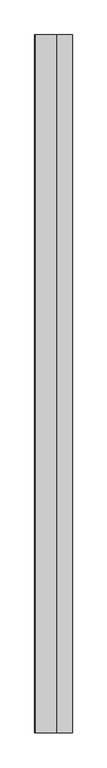
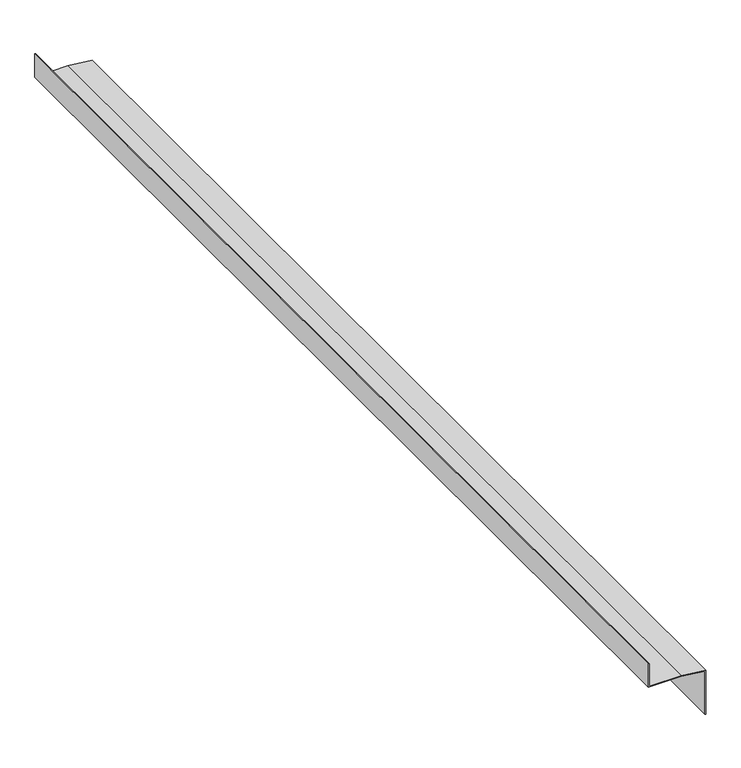
"""IFC4 building model written with IfcOpenShell, lengths in millimetres: proxy geometry, Generic Models 7:Generic Models 1:7:Generic Models 1:7 : Generic Models 7:Generic Models 1:337419:8 : Generic Models 7:Generic Models 1:7:Generic Models 1:7 : Generic Models 7:Generic Models 1:337419:315055."""

from ifc_helpers import new_model, si_unit, frame, origin, place, context, project, spatial, polyline, outline, extrude, source, transform, mapped, element, save


def generic_models_aac07dfa(model_context):
    return source(origin(), model_context, "Body", "SweptSolid", [
        extrude(outline(polyline([(-1.5875, 0.0), (0.0, 0.0), (0.0, -106.0492371), (-55.4288014, -112.2039841), (-129.4872829, -112.2039841), (-129.4872829, -167.5335098), (-131.0747829, -167.5335098), (-131.0747829, -110.6164841), (-55.5166684, -110.6164841), (-1.5875, -104.6282546), (-1.5875, 0.0)])), frame((667691.4364106, -507639.2545751, -81.7582633), z_axis=(1.6692203175239229e-12, 1.0, 0.0), x_axis=(1.0, -1.6692203175239229e-12, 0.0)), (0.0, 0.0, 1.0), 2431.2755388),
    ])


if __name__ == "__main__":
    model = new_model("IFC4")
    model_context = context("Model", 3, world=origin())
    ifc_project = project(units=[si_unit("LENGTHUNIT", "METRE", prefix="MILLI")], contexts=[model_context])
    site = spatial("IfcSite", under=ifc_project)
    building = spatial("IfcBuilding", under=site)
    placement = place(None, origin())
    generic_models_shape = generic_models_aac07dfa(model_context)
    element("IfcBuildingElementProxy", 1, Name="Generic Models 7:Generic Models 1:7:Generic Models 1:7 : Generic Models 7:Generic Models 1:337419:8 : Generic Models 7:Generic Models 1:7:Generic Models 1:7 : Generic Models 7:Generic Models 1:337419:315055", ObjectType="Generic Models 7:Generic Models 1:7:Generic Models 1:7 : Generic Models 7:Generic Models 1:337419:8 : Generic Models 7:Generic Models 1:7:Generic Models 1:7 : Generic Models 7:Generic Models 1:337419:315055", at=placement, inside=building, context=model_context, shape_type="MappedRepresentation", body=[
        mapped(generic_models_shape, transform((0.0, 0.0, 0.0), x_axis=(1.0, 0.0, 0.0), y_axis=(0.0, 1.0, 0.0), z_axis=(0.0, 0.0, 1.0))),
    ])
    save(model, "model.ifc")

# Revit data of these elements
# Type "Generic Models 7:Generic Models 1:7:Generic Models 1:7 : Generic Models 7:Generic Models 1:337419:8 : Generic Models 7:Generic Models 1:7:Generic Models 1:7 : Generic Models 7:Generic Models 1:337419:315055"
#   NameOverride = "Generic Models 7:Generic Models 1:7:Generic Models 1:7 : Generic Models 7:Generic Models 1:337419:315055"
#   ObjectTypeOverride = "Generic Models 1:7 : Generic Models 7:Generic Models 1:337419"
#   Reference = "Generic Models 1"
#   Tag = "315055"
# Element 1 (IfcBuildingElementProxy, "Generic Models 7:Generic Models 1:7:Generic Models 1:7 : Generic Models 7:Generic Models 1:337419:8 : Generic Models 7:Generic Models 1:7:Generic Models 1:7 : Generic Models 7:Generic Models 1:337419:315055")
#   Materials on its faces: "ANODIZED ALUM. FLASHING - MATCH STOREFRONT (ALIGN WITH OTHER WALL ASSEMBLIES)"
# Materials
#   "ANODIZED ALUM. FLASHING - MATCH STOREFRONT (ALIGN WITH OTHER WALL ASSEMBLIES)": class "Unassigned", colour RGB 210 209 208, transparency 0, Cost = 0
